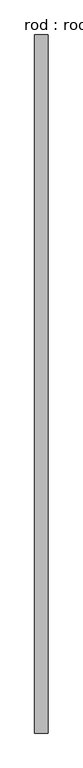
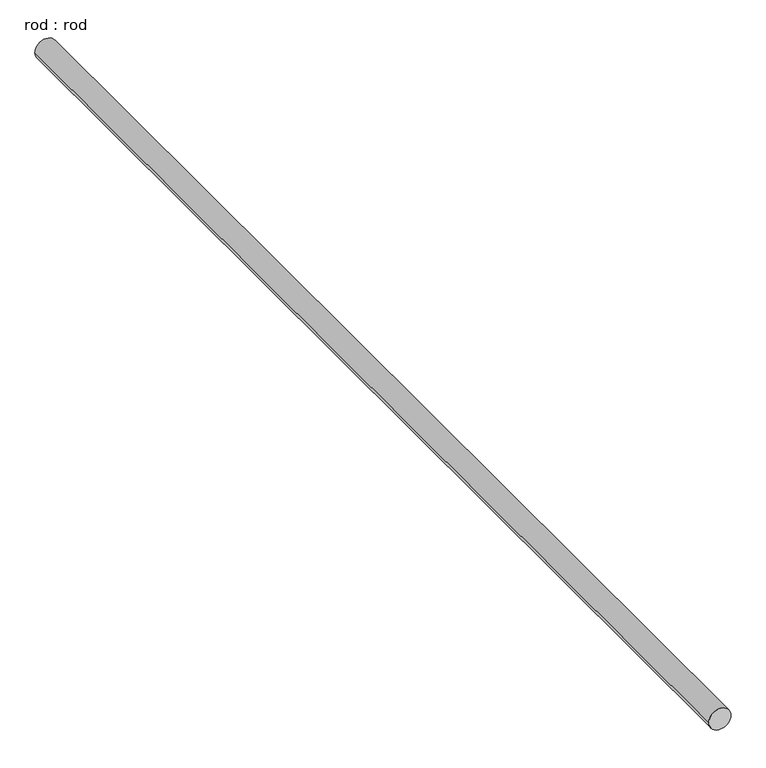
"""IFC4 building model written with IfcOpenShell, lengths in millimetres: proxy geometry, rod : rod."""

from ifc_helpers import new_model, si_unit, point, frame, frame_2d, origin, place, context, project, spatial, circle_curve, trimmed, segment, composite_curve, outline, extrude, source, transform, mapped, element, save


def rod_rod_11387980(model_context):
    return source(origin(), model_context, "Body", "SweptSolid", [
        extrude(outline(composite_curve([segment(trimmed(circle_curve(frame_2d((0.0108462, 0.0)), 200.0), [point((0.0108462, 200.0))], [point((0.0108462, -200.0))], False, "CARTESIAN"), True, "CONTINUOUS"), segment(trimmed(circle_curve(frame_2d((0.0108462, 0.0)), 200.0), [point((0.0108462, -200.0))], [point((0.0108462, 200.0))], False, "CARTESIAN"), True, "CONTINUOUS")], self_intersect=False)), frame((0.0, -6464.8195767, 0.0), z_axis=(0.0, 1.0, 0.0), x_axis=(0.0, 0.0, 1.0)), (0.0, 0.0, 1.0), 21115.0963842),
    ])


if __name__ == "__main__":
    model = new_model("IFC4")
    model_context = context("Model", 3, world=origin())
    ifc_project = project(units=[si_unit("LENGTHUNIT", "METRE", prefix="MILLI")], contexts=[model_context])
    site = spatial("IfcSite", under=ifc_project)
    building = spatial("IfcBuilding", under=site)
    placement = place(None, origin())
    rod_rod_shape = rod_rod_11387980(model_context)
    element("IfcBuildingElementProxy", 1, Name="rod : rod", ObjectType="rod : rod", at=placement, inside=building, context=model_context, shape_type="MappedRepresentation", body=[
        mapped(rod_rod_shape, transform((0.0, 0.0, 0.0), x_axis=(1.0, 0.0, 0.0), y_axis=(0.0, 1.0, 0.0), z_axis=(0.0, 0.0, 1.0))),
    ])
    save(model, "model.ifc")

# Revit data of these elements
# Type "rod : rod"
#   Default Elevation = 0
